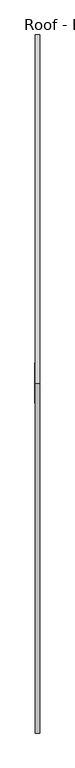
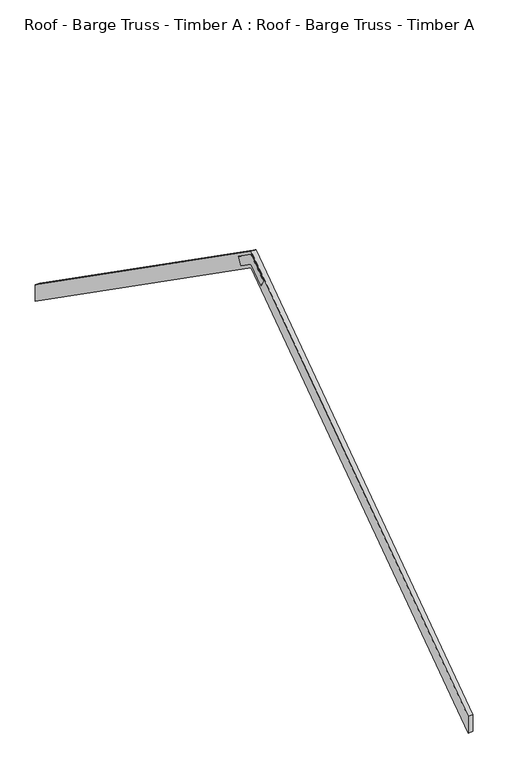
"""IFC4 building model written with IfcOpenShell, lengths in millimetres: furniture geometry, Roof - Barge Truss - Timber A : Roof - Barge Truss - Timber A."""

import ifcopenshell
import ifcopenshell.guid

model = None  # the IFC model being written
_history = None  # IfcOwnerHistory: only IFC2X3 demands one
_inside = {}  # id of a spatial element -> (the spatial element, [elements in it])
_under = {}  # id of a project, library or spatial element -> (it, [spatial elements below it])
_declared = {}  # id of a project -> (the project, [libraries it declares])
_typed = {}  # id of a type object -> (the type object, [elements of that type])
_made_of = {}  # id of a material, layer set ... -> (it, [elements and type objects made of it])


def new_model(schema):
    """Start an empty IFC model of exactly this schema.

    Asked for "IFC4X3", IfcOpenShell would pick the latest addendum, in which some entities
    have other attributes; the version numbers below select the first issue.
    IFC2X3 requires an IfcOwnerHistory on every rooted entity: one is made here for all.
    """
    global model, _history
    if schema == "IFC4X3":
        model = ifcopenshell.file(schema_version=(4, 3, 0, 0))
    else:
        model = ifcopenshell.file(schema=schema)
    _inside.clear()
    _under.clear()
    _declared.clear()
    _typed.clear()
    _made_of.clear()
    _history = None
    if model.schema == "IFC2X3":
        org = make("IfcOrganization", Name="unknown")
        user = make(
            "IfcPersonAndOrganization",
            ThePerson=make("IfcPerson", FamilyName="unknown"),
            TheOrganization=org,
        )
        app = make(
            "IfcApplication",
            ApplicationDeveloper=org,
            Version="unknown",
            ApplicationFullName="unknown",
            ApplicationIdentifier="unknown",
        )
        _history = make(
            "IfcOwnerHistory",
            OwningUser=user,
            OwningApplication=app,
            ChangeAction="ADDED",
            CreationDate=0,
        )
    return model


def make(cls, **values):
    """One entity of the class cls with the attributes given. An attribute that is None is left unset."""
    return model.create_entity(
        cls, **{name: value for name, value in values.items() if value is not None}
    )


def rooted(cls, **values):
    """An entity with a GlobalId (a new one), such as an element, a storey or a relation."""
    return make(cls, GlobalId=ifcopenshell.guid.new(), OwnerHistory=_history, **values)


def si_unit(unit_type, name, prefix=None):
    """IfcSIUnit, for example si_unit("LENGTHUNIT", "METRE", prefix="MILLI")."""
    return make("IfcSIUnit", UnitType=unit_type, Prefix=prefix, Name=name)


def assignment(units):
    """IfcUnitAssignment: the units of a project."""
    return None if units is None else make("IfcUnitAssignment", Units=units)


def point(xyz):
    """IfcCartesianPoint."""
    return None if xyz is None else make("IfcCartesianPoint", Coordinates=xyz)


def direction(xyz):
    """IfcDirection."""
    return None if xyz is None else make("IfcDirection", DirectionRatios=xyz)


def frame(location, z_axis=None, x_axis=None):
    """IfcAxis2Placement3D, a coordinate frame: its origin and axes. An axis left out is left unset."""
    return make(
        "IfcAxis2Placement3D",
        Location=point(location),
        Axis=direction(z_axis),
        RefDirection=direction(x_axis),
    )


def origin():
    """The frame at (0, 0, 0) with its axes left unset."""
    return frame((0.0, 0.0, 0.0))


def place(relative_to, where):
    """IfcLocalPlacement: puts the frame where relative to a parent placement (None: the world)."""
    return make(
        "IfcLocalPlacement", PlacementRelTo=relative_to, RelativePlacement=where
    )


def context(
    kind, dimensions, precision=None, world=None, true_north=None, identifier=None
):
    """IfcGeometricRepresentationContext, for example the 3D "Model" context."""
    return make(
        "IfcGeometricRepresentationContext",
        ContextIdentifier=identifier,
        ContextType=kind,
        CoordinateSpaceDimension=dimensions,
        Precision=precision,
        WorldCoordinateSystem=world,
        TrueNorth=true_north,
    )


def project(units=None, contexts=None):
    """IfcProject with its units and contexts."""
    return rooted(
        "IfcProject",
        Name="project",
        RepresentationContexts=contexts,
        UnitsInContext=assignment(units),
    )


def spatial(cls, under=None, at=None, **own):
    """A site, building, storey or space (cls), placed at a placement, below another one or the project."""
    s = rooted(cls, ObjectPlacement=at, **own)
    if under is not None:
        _under.setdefault(under.id(), (under, []))[1].append(s)
    return s


def polyline(points):
    """IfcPolyline through the points."""
    return make("IfcPolyline", Points=[point(p) for p in points])


def outline(outer, holes=None, kind="AREA"):
    """IfcArbitraryClosedProfileDef: a profile drawn as a closed curve; with holes, ...WithVoids."""
    if holes is None:
        return make("IfcArbitraryClosedProfileDef", ProfileType=kind, OuterCurve=outer)
    return make(
        "IfcArbitraryProfileDefWithVoids",
        ProfileType=kind,
        OuterCurve=outer,
        InnerCurves=holes,
    )


def extrude(swept, where, along, depth):
    """IfcExtrudedAreaSolid: the profile swept, set in the frame where, extruded along a direction by depth."""
    return make(
        "IfcExtrudedAreaSolid",
        SweptArea=swept,
        Position=where,
        ExtrudedDirection=direction(along),
        Depth=depth,
    )


def shape(context_of_items, identifier, shape_type, items):
    """IfcShapeRepresentation: the items that make up one representation, for example the "Body"."""
    return make(
        "IfcShapeRepresentation",
        ContextOfItems=context_of_items,
        RepresentationIdentifier=identifier,
        RepresentationType=shape_type,
        Items=items,
    )


def source(mapping_origin, context_of_items, identifier, shape_type, items):
    """IfcRepresentationMap: a shape defined once, which mapped items show again and again."""
    return make(
        "IfcRepresentationMap",
        MappingOrigin=mapping_origin,
        MappedRepresentation=shape(context_of_items, identifier, shape_type, items),
    )


def transform(
    local_origin,
    x_axis=None,
    y_axis=None,
    z_axis=None,
    scale=None,
    scale2=None,
    scale3=None,
    uniform=True,
):
    """IfcCartesianTransformationOperator3D, or its non-uniform kind. x_axis, y_axis, z_axis: its Axis1, 2, 3."""
    if uniform:
        return make(
            "IfcCartesianTransformationOperator3D",
            Axis1=direction(x_axis),
            Axis2=direction(y_axis),
            LocalOrigin=point(local_origin),
            Scale=scale,
            Axis3=direction(z_axis),
        )
    return make(
        "IfcCartesianTransformationOperator3DnonUniform",
        Axis1=direction(x_axis),
        Axis2=direction(y_axis),
        LocalOrigin=point(local_origin),
        Scale=scale,
        Axis3=direction(z_axis),
        Scale2=scale2,
        Scale3=scale3,
    )


def mapped(mapping_source, mapping_target):
    """IfcMappedItem: shows the shape of a source again, moved by a transform."""
    return make(
        "IfcMappedItem", MappingSource=mapping_source, MappingTarget=mapping_target
    )


def made_of(thing, what):
    """Note that an element or type object is made of a material, layer set ...; save() writes the relation."""
    if what is not None:
        _made_of.setdefault(what.id(), (what, []))[1].append(thing)
    return thing


def element(
    cls,
    number,
    at=None,
    inside=None,
    cuts=None,
    type_object=None,
    material=None,
    context=None,
    identifier="Body",
    shape_type=None,
    held_by="IfcProductDefinitionShape",
    body=None,
    shapes=None,
    **own,
):
    """One element of the class cls, such as IfcWall. Its Tag is "e" and its number.

    at: its placement. inside: the storey or other place that contains it. cuts: it is an
    opening in that element (IfcRelVoidsElement). A single representation is given by context,
    identifier, shape_type and body (its items); several are given by shapes. held_by: the class
    of the entity that holds the representations. save() writes the other relations.
    """
    e = rooted(cls, Tag="e%d" % number, ObjectPlacement=at, **own)
    if body is not None:
        shapes = [shape(context, identifier, shape_type, body)]
    if shapes is not None:
        e.Representation = make(held_by, Representations=shapes)
    if inside is not None:
        _inside.setdefault(inside.id(), (inside, []))[1].append(e)
    if cuts is not None:
        rooted(
            "IfcRelVoidsElement", RelatingBuildingElement=cuts, RelatedOpeningElement=e
        )
    if type_object is not None:
        _typed.setdefault(type_object.id(), (type_object, []))[1].append(e)
    return made_of(e, material)


def aggregate(whole, parts):
    """IfcRelAggregates: a whole, such as a stair, and the parts it consists of."""
    return rooted("IfcRelAggregates", RelatingObject=whole, RelatedObjects=parts)


def save(model, path):
    """Write the relations noted so far, then the file.

    IfcRelAggregates (storeys below a building ...), IfcRelContainedInSpatialStructure (elements
    in a storey), IfcRelDefinesByType, IfcRelAssociatesMaterial and IfcRelDeclares: one each for
    every whole, place, type object, material and project.
    """
    for whole, parts in _under.values():
        aggregate(whole, parts)
    for where, things in _inside.values():
        rooted(
            "IfcRelContainedInSpatialStructure",
            RelatedElements=things,
            RelatingStructure=where,
        )
    for kind, things in _typed.values():
        rooted("IfcRelDefinesByType", RelatedObjects=things, RelatingType=kind)
    for what, things in _made_of.values():
        rooted("IfcRelAssociatesMaterial", RelatedObjects=things, RelatingMaterial=what)
    for by, libraries in _declared.values():
        rooted("IfcRelDeclares", RelatingContext=by, RelatedDefinitions=libraries)
    model.write(path)


def roof_barge_truss_timber_a_roof_barge_truss_timber_a_2ed991f7(model_context):
    return source(origin(), model_context, "Body", "SweptSolid", [
        extrude(outline(polyline([(-300.0, 2810.9005033), (3620.25, 65.9119017), (3620.25, -117.2042867), (-300.0, 2627.784315), (-4239.4775971, -130.6675951), (-4239.4775971, 52.4485932), (-300.0, 2810.9005033)])), frame((19.8827307, 0.0, 0.0), z_axis=(1.0, 0.0, 0.0), x_axis=(0.0, 1.0, 0.0)), (0.0, 0.0, 1.0), 49.6351915),
        extrude(outline(polyline([(-299.7806483, 2778.8151222), (-72.8793639, 2619.9371325), (-119.3123526, 2542.6596622), (-299.7238694, 2668.9851662), (-480.2153155, 2542.6036951), (-526.6819326, 2619.9371325), (-299.7806483, 2778.8151222)])), frame((17.4104988, 0.0, 0.0), z_axis=(1.0, 0.0, 0.0), x_axis=(0.0, 1.0, 0.0)), (0.0, 0.0, 1.0), 2.4722319),
        extrude(outline(polyline([(-299.7806483, 2777.9554848), (-72.8793639, 2619.0774951), (-119.345981, 2541.7440577), (-299.7806483, 2668.0857719), (-480.2153155, 2541.7440577), (-526.6819326, 2619.0774951), (-299.7806483, 2777.9554848)])), frame((69.5179222, 0.0, 0.0), z_axis=(1.0, 0.0, 0.0), x_axis=(0.0, 1.0, 0.0)), (0.0, 0.0, 1.0), 2.0827493),
    ])


if __name__ == "__main__":
    model = new_model("IFC4")
    model_context = context("Model", 3, world=origin())
    ifc_project = project(units=[si_unit("LENGTHUNIT", "METRE", prefix="MILLI")], contexts=[model_context])
    site = spatial("IfcSite", under=ifc_project)
    building = spatial("IfcBuilding", under=site)
    placement = place(None, origin())
    roof_barge_truss_timber_a_roof_barge_truss_timber_a_shape = roof_barge_truss_timber_a_roof_barge_truss_timber_a_2ed991f7(model_context)
    element("IfcFurniture", 1, ObjectType="Roof - Barge Truss - Timber A : Roof - Barge Truss - Timber A", at=placement, inside=building, context=model_context, shape_type="MappedRepresentation", body=[
        mapped(roof_barge_truss_timber_a_roof_barge_truss_timber_a_shape, transform((0.0, 0.0, 0.0), x_axis=(1.0, 0.0, 0.0), y_axis=(0.0, 1.0, 0.0), z_axis=(0.0, 0.0, 1.0))),
    ])
    save(model, "model.ifc")

# Revit data of these elements
# Type "Roof - Barge Truss - Timber A : Roof - Barge Truss - Timber A"
#   Manufacturer = "M W Roofs"
#   Finish = "Rough"
#   Description = "Preformed Gangnail Barge ladder Truss"
#   Construction Type = "Timber"
#   Depth = 600 mm
#   Height = 900 mm
#   Width = 900 mm
#   Default Elevation = 0
# Element 1 (IfcFurniture, "Roof - Barge Truss - Timber A : Roof - Barge Truss - Timber A")
#   Materials on its faces: "Softwood, Lumber"
# Materials
#   "Softwood, Lumber": class "Wood", colour RGB 205 156 65, transparency 0, Description = "Pinus Echinata", Cost = 0
